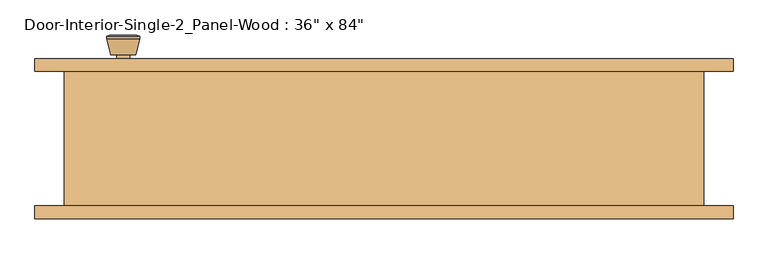
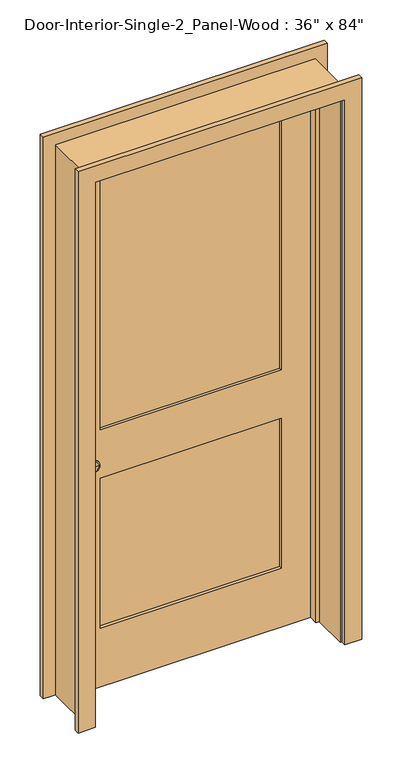
"""IFC4 building model written with IfcOpenShell, lengths in millimetres: door geometry."""

import ifcopenshell
import ifcopenshell.guid

model = None  # the IFC model being written
_history = None  # IfcOwnerHistory: only IFC2X3 demands one
_inside = {}  # id of a spatial element -> (the spatial element, [elements in it])
_under = {}  # id of a project, library or spatial element -> (it, [spatial elements below it])
_declared = {}  # id of a project -> (the project, [libraries it declares])
_typed = {}  # id of a type object -> (the type object, [elements of that type])
_made_of = {}  # id of a material, layer set ... -> (it, [elements and type objects made of it])


def new_model(schema):
    """Start an empty IFC model of exactly this schema.

    Asked for "IFC4X3", IfcOpenShell would pick the latest addendum, in which some entities
    have other attributes; the version numbers below select the first issue.
    IFC2X3 requires an IfcOwnerHistory on every rooted entity: one is made here for all.
    """
    global model, _history
    if schema == "IFC4X3":
        model = ifcopenshell.file(schema_version=(4, 3, 0, 0))
    else:
        model = ifcopenshell.file(schema=schema)
    _inside.clear()
    _under.clear()
    _declared.clear()
    _typed.clear()
    _made_of.clear()
    _history = None
    if model.schema == "IFC2X3":
        org = make("IfcOrganization", Name="unknown")
        user = make(
            "IfcPersonAndOrganization",
            ThePerson=make("IfcPerson", FamilyName="unknown"),
            TheOrganization=org,
        )
        app = make(
            "IfcApplication",
            ApplicationDeveloper=org,
            Version="unknown",
            ApplicationFullName="unknown",
            ApplicationIdentifier="unknown",
        )
        _history = make(
            "IfcOwnerHistory",
            OwningUser=user,
            OwningApplication=app,
            ChangeAction="ADDED",
            CreationDate=0,
        )
    return model


def make(cls, **values):
    """One entity of the class cls with the attributes given. An attribute that is None is left unset."""
    return model.create_entity(
        cls, **{name: value for name, value in values.items() if value is not None}
    )


def rooted(cls, **values):
    """An entity with a GlobalId (a new one), such as an element, a storey or a relation."""
    return make(cls, GlobalId=ifcopenshell.guid.new(), OwnerHistory=_history, **values)


def si_unit(unit_type, name, prefix=None):
    """IfcSIUnit, for example si_unit("LENGTHUNIT", "METRE", prefix="MILLI")."""
    return make("IfcSIUnit", UnitType=unit_type, Prefix=prefix, Name=name)


def assignment(units):
    """IfcUnitAssignment: the units of a project."""
    return None if units is None else make("IfcUnitAssignment", Units=units)


def point(xyz):
    """IfcCartesianPoint."""
    return None if xyz is None else make("IfcCartesianPoint", Coordinates=xyz)


def direction(xyz):
    """IfcDirection."""
    return None if xyz is None else make("IfcDirection", DirectionRatios=xyz)


def frame(location, z_axis=None, x_axis=None):
    """IfcAxis2Placement3D, a coordinate frame: its origin and axes. An axis left out is left unset."""
    return make(
        "IfcAxis2Placement3D",
        Location=point(location),
        Axis=direction(z_axis),
        RefDirection=direction(x_axis),
    )


def frame_2d(location, x_axis=None):
    """IfcAxis2Placement2D, a coordinate frame in the plane: its origin and x axis."""
    return make(
        "IfcAxis2Placement2D", Location=point(location), RefDirection=direction(x_axis)
    )


def origin():
    """The frame at (0, 0, 0) with its axes left unset."""
    return frame((0.0, 0.0, 0.0))


def place(relative_to, where):
    """IfcLocalPlacement: puts the frame where relative to a parent placement (None: the world)."""
    return make(
        "IfcLocalPlacement", PlacementRelTo=relative_to, RelativePlacement=where
    )


def context(
    kind, dimensions, precision=None, world=None, true_north=None, identifier=None
):
    """IfcGeometricRepresentationContext, for example the 3D "Model" context."""
    return make(
        "IfcGeometricRepresentationContext",
        ContextIdentifier=identifier,
        ContextType=kind,
        CoordinateSpaceDimension=dimensions,
        Precision=precision,
        WorldCoordinateSystem=world,
        TrueNorth=true_north,
    )


def project(units=None, contexts=None):
    """IfcProject with its units and contexts."""
    return rooted(
        "IfcProject",
        Name="project",
        RepresentationContexts=contexts,
        UnitsInContext=assignment(units),
    )


def spatial(cls, under=None, at=None, **own):
    """A site, building, storey or space (cls), placed at a placement, below another one or the project."""
    s = rooted(cls, ObjectPlacement=at, **own)
    if under is not None:
        _under.setdefault(under.id(), (under, []))[1].append(s)
    return s


def polyline(points):
    """IfcPolyline through the points."""
    return make("IfcPolyline", Points=[point(p) for p in points])


def circle_curve(where, radius):
    """IfcCircle in the frame where."""
    return make("IfcCircle", Position=where, Radius=radius)


def trimmed(basis, trim1, trim2, sense, master):
    """IfcTrimmedCurve: the piece of a basis curve between two trims."""
    return make(
        "IfcTrimmedCurve",
        BasisCurve=basis,
        Trim1=trim1,
        Trim2=trim2,
        SenseAgreement=sense,
        MasterRepresentation=master,
    )


def segment(curve, same_sense, transition):
    """IfcCompositeCurveSegment."""
    return make(
        "IfcCompositeCurveSegment",
        Transition=transition,
        SameSense=same_sense,
        ParentCurve=curve,
    )


def composite_curve(segments, self_intersect=None):
    """IfcCompositeCurve: segments joined end to end."""
    return make("IfcCompositeCurve", Segments=segments, SelfIntersect=self_intersect)


def outline(outer, holes=None, kind="AREA"):
    """IfcArbitraryClosedProfileDef: a profile drawn as a closed curve; with holes, ...WithVoids."""
    if holes is None:
        return make("IfcArbitraryClosedProfileDef", ProfileType=kind, OuterCurve=outer)
    return make(
        "IfcArbitraryProfileDefWithVoids",
        ProfileType=kind,
        OuterCurve=outer,
        InnerCurves=holes,
    )


def extrude(swept, where, along, depth):
    """IfcExtrudedAreaSolid: the profile swept, set in the frame where, extruded along a direction by depth."""
    return make(
        "IfcExtrudedAreaSolid",
        SweptArea=swept,
        Position=where,
        ExtrudedDirection=direction(along),
        Depth=depth,
    )


def faces_of(points, faces, orient=None, outer=None):
    """IfcFace entities. A face is a list of loops; a loop is a list of indices into points, from 0.

    orient and outer hold one flag for each loop. By default every Orientation is true, the
    first loop of a face is its IfcFaceOuterBound and the others are IfcFaceBound.
    """
    made = []
    for i, loops in enumerate(faces):
        bounds = []
        for j, loop in enumerate(loops):
            is_outer = j == 0 if outer is None else outer[i][j]
            bounds.append(
                make(
                    "IfcFaceOuterBound" if is_outer else "IfcFaceBound",
                    Bound=make("IfcPolyLoop", Polygon=[points[k] for k in loop]),
                    Orientation=True if orient is None else orient[i][j],
                )
            )
        made.append(make("IfcFace", Bounds=bounds))
    return made


def faceted_brep(points, faces, orient=None, outer=None, voids=None):
    """IfcFacetedBrep: a solid bounded by flat faces; with voids (closed shells), ...WithVoids."""
    shared = [point(p) for p in points]
    hull = make("IfcClosedShell", CfsFaces=faces_of(shared, faces, orient, outer))
    if voids is None:
        return make("IfcFacetedBrep", Outer=hull)
    return make(
        "IfcFacetedBrepWithVoids",
        Outer=hull,
        Voids=[
            make(cls, CfsFaces=faces_of(shared, fs, o, b)) for cls, fs, o, b in voids
        ],
    )


def shape(context_of_items, identifier, shape_type, items):
    """IfcShapeRepresentation: the items that make up one representation, for example the "Body"."""
    return make(
        "IfcShapeRepresentation",
        ContextOfItems=context_of_items,
        RepresentationIdentifier=identifier,
        RepresentationType=shape_type,
        Items=items,
    )


def source(mapping_origin, context_of_items, identifier, shape_type, items):
    """IfcRepresentationMap: a shape defined once, which mapped items show again and again."""
    return make(
        "IfcRepresentationMap",
        MappingOrigin=mapping_origin,
        MappedRepresentation=shape(context_of_items, identifier, shape_type, items),
    )


def transform(
    local_origin,
    x_axis=None,
    y_axis=None,
    z_axis=None,
    scale=None,
    scale2=None,
    scale3=None,
    uniform=True,
):
    """IfcCartesianTransformationOperator3D, or its non-uniform kind. x_axis, y_axis, z_axis: its Axis1, 2, 3."""
    if uniform:
        return make(
            "IfcCartesianTransformationOperator3D",
            Axis1=direction(x_axis),
            Axis2=direction(y_axis),
            LocalOrigin=point(local_origin),
            Scale=scale,
            Axis3=direction(z_axis),
        )
    return make(
        "IfcCartesianTransformationOperator3DnonUniform",
        Axis1=direction(x_axis),
        Axis2=direction(y_axis),
        LocalOrigin=point(local_origin),
        Scale=scale,
        Axis3=direction(z_axis),
        Scale2=scale2,
        Scale3=scale3,
    )


def mapped(mapping_source, mapping_target):
    """IfcMappedItem: shows the shape of a source again, moved by a transform."""
    return make(
        "IfcMappedItem", MappingSource=mapping_source, MappingTarget=mapping_target
    )


def made_of(thing, what):
    """Note that an element or type object is made of a material, layer set ...; save() writes the relation."""
    if what is not None:
        _made_of.setdefault(what.id(), (what, []))[1].append(thing)
    return thing


def element(
    cls,
    number,
    at=None,
    inside=None,
    cuts=None,
    type_object=None,
    material=None,
    context=None,
    identifier="Body",
    shape_type=None,
    held_by="IfcProductDefinitionShape",
    body=None,
    shapes=None,
    **own,
):
    """One element of the class cls, such as IfcWall. Its Tag is "e" and its number.

    at: its placement. inside: the storey or other place that contains it. cuts: it is an
    opening in that element (IfcRelVoidsElement). A single representation is given by context,
    identifier, shape_type and body (its items); several are given by shapes. held_by: the class
    of the entity that holds the representations. save() writes the other relations.
    """
    e = rooted(cls, Tag="e%d" % number, ObjectPlacement=at, **own)
    if body is not None:
        shapes = [shape(context, identifier, shape_type, body)]
    if shapes is not None:
        e.Representation = make(held_by, Representations=shapes)
    if inside is not None:
        _inside.setdefault(inside.id(), (inside, []))[1].append(e)
    if cuts is not None:
        rooted(
            "IfcRelVoidsElement", RelatingBuildingElement=cuts, RelatedOpeningElement=e
        )
    if type_object is not None:
        _typed.setdefault(type_object.id(), (type_object, []))[1].append(e)
    return made_of(e, material)


def aggregate(whole, parts):
    """IfcRelAggregates: a whole, such as a stair, and the parts it consists of."""
    return rooted("IfcRelAggregates", RelatingObject=whole, RelatedObjects=parts)


def save(model, path):
    """Write the relations noted so far, then the file.

    IfcRelAggregates (storeys below a building ...), IfcRelContainedInSpatialStructure (elements
    in a storey), IfcRelDefinesByType, IfcRelAssociatesMaterial and IfcRelDeclares: one each for
    every whole, place, type object, material and project.
    """
    for whole, parts in _under.values():
        aggregate(whole, parts)
    for where, things in _inside.values():
        rooted(
            "IfcRelContainedInSpatialStructure",
            RelatedElements=things,
            RelatingStructure=where,
        )
    for kind, things in _typed.values():
        rooted("IfcRelDefinesByType", RelatedObjects=things, RelatingType=kind)
    for what, things in _made_of.values():
        rooted("IfcRelAssociatesMaterial", RelatedObjects=things, RelatingMaterial=what)
    for by, libraries in _declared.values():
        rooted("IfcRelDeclares", RelatingContext=by, RelatedDefinitions=libraries)
    model.write(path)


def plane_surface(at):
    """IfcPlane: the flat surface through the origin of the frame at, square to its z axis."""
    return make("IfcPlane", Position=at)


def cylinder_surface(at, radius):
    """IfcCylindricalSurface: all points at the distance radius from the z axis of the frame at."""
    return make("IfcCylindricalSurface", Position=at, Radius=radius)


def revolved_surface(curve, axis_point, axis_direction):
    """IfcSurfaceOfRevolution: the curve turned about the line through axis_point along axis_direction."""
    return make(
        "IfcSurfaceOfRevolution",
        SweptCurve=make("IfcArbitraryOpenProfileDef", ProfileType="CURVE", Curve=curve),
        AxisPosition=make("IfcAxis1Placement", Location=point(axis_point), Axis=direction(axis_direction)),
    )


def advanced_brep(points, edges, surfaces, faces):
    """IfcAdvancedBrep: a solid bounded by faces that lie on surfaces and meet in shared edges.

    An edge is (start, end): straight between two places in points (the first is 0);
    or (start, end, curve); or (start, end, curve, False) where it runs against its curve.
    A face is (place in surfaces, loops), or (place, loops, False) where it looks against
    its surface's normal. A loop lists edges by number (the first is 1), with a minus sign
    where the edge is run from its end to its start. The first loop is the outer one.
    """
    corners = [point(p) for p in points]
    vertices = [make("IfcVertexPoint", VertexGeometry=c) for c in corners]
    made = []
    for start, end, *more in edges:
        made.append(
            make(
                "IfcEdgeCurve",
                EdgeStart=vertices[start],
                EdgeEnd=vertices[end],
                EdgeGeometry=more[0] if more else make("IfcPolyline", Points=[corners[start], corners[end]]),
                SameSense=more[1] if len(more) > 1 else True,
            )
        )
    hull = []
    for where, loops, *sense in faces:
        bounds = []
        for j, loop in enumerate(loops):
            ring = [make("IfcOrientedEdge", EdgeElement=made[abs(k) - 1], Orientation=k > 0) for k in loop]
            bounds.append(
                make(
                    "IfcFaceOuterBound" if j == 0 else "IfcFaceBound",
                    Bound=make("IfcEdgeLoop", EdgeList=ring),
                    Orientation=True,
                )
            )
        hull.append(make("IfcAdvancedFace", Bounds=bounds, FaceSurface=surfaces[where], SameSense=sense[0] if sense else True))
    return make("IfcAdvancedBrep", Outer=make("IfcClosedShell", CfsFaces=hull))


def door_6f959a6d(model_context):
    return source(origin(), model_context, "Body", "SolidModel", [
        advanced_brep(
        [(-393.7, 57.5, 914.4), (-383.7, 57.5, 914.4), (-403.7, 57.5, 914.4), (-373.2241324, 8.5, 914.4), (-393.7, 8.5, 914.4), (-414.1758676, 8.5, 914.4), (-368.7, 10.3278681, 914.4), (-418.7, 10.3278681, 914.4), (-368.7, 13.7915463, 914.4), (-418.7, 13.7915463, 914.4), (-375.063764, 38.5, 914.4), (-412.336236, 38.5, 914.4), (-383.7, 38.5, 914.4), (-403.7, 38.5, 914.4)],
        [
            (0, 1),
            (1, 2, circle_curve(frame((-393.7, 57.5, 914.4), z_axis=(0.0, 1.0, 0.0), x_axis=(-1.0, 0.0, 0.0)), 10.0)),
            (2, 0),
            (2, 1, circle_curve(frame((-393.7, 57.5, 914.4), z_axis=(0.0, 1.0, 0.0), x_axis=(-1.0, 0.0, 0.0)), 10.0)),
            (3, 4),
            (4, 5),
            (5, 3, circle_curve(frame((-393.7, 8.5, 914.4), z_axis=(0.0, -1.0, 0.0), x_axis=(-1.0, 0.0, 0.0)), 20.4758676)),
            (3, 5, circle_curve(frame((-393.7, 8.5, 914.4), z_axis=(0.0, -1.0, 0.0), x_axis=(-1.0, 0.0, 0.0)), 20.4758676)),
            (6, 3),
            (5, 7),
            (7, 6, circle_curve(frame((-393.7, 10.3278681, 914.4), z_axis=(0.0, -1.0, 0.0), x_axis=(-1.0, 0.0, 0.0)), 25.0)),
            (6, 7, circle_curve(frame((-393.7, 10.3278681, 914.4), z_axis=(0.0, -1.0, 0.0), x_axis=(-1.0, 0.0, 0.0)), 25.0)),
            (8, 6),
            (7, 9),
            (9, 8, circle_curve(frame((-393.7, 13.7915463, 914.4), z_axis=(0.0, -1.0, 0.0), x_axis=(-1.0, 0.0, 0.0)), 25.0)),
            (8, 9, circle_curve(frame((-393.7, 13.7915463, 914.4), z_axis=(0.0, -1.0, 0.0), x_axis=(-1.0, 0.0, 0.0)), 25.0)),
            (10, 8),
            (9, 11),
            (11, 10, circle_curve(frame((-393.7, 38.5, 914.4), z_axis=(0.0, -1.0, 0.0), x_axis=(-1.0, 0.0, 0.0)), 18.636236)),
            (10, 11, circle_curve(frame((-393.7, 38.5, 914.4), z_axis=(0.0, -1.0, 0.0), x_axis=(-1.0, 0.0, 0.0)), 18.636236)),
            (12, 10),
            (11, 13),
            (13, 12, circle_curve(frame((-393.7, 38.5, 914.4), z_axis=(0.0, -1.0, 0.0), x_axis=(-1.0, 0.0, 0.0)), 10.0)),
            (12, 13, circle_curve(frame((-393.7, 38.5, 914.4), z_axis=(0.0, -1.0, 0.0), x_axis=(-1.0, 0.0, 0.0)), 10.0)),
            (1, 12),
            (13, 2),
        ],
        [
            plane_surface(frame((-393.7, 57.5, 914.4), z_axis=(0.0, 1.0, 0.0), x_axis=(-1.0, 0.0, 0.0))),
            plane_surface(frame((-393.7, 8.5, 914.4), z_axis=(0.0, -1.0, 0.0), x_axis=(-1.0, 0.0, 0.0))),
            revolved_surface(polyline([(-414.1758676, 8.5, 914.4), (-418.7, 10.3278681, 914.4)]), (-393.7, 57.5, 914.4), (0.0, 1.0, 0.0)),
            cylinder_surface(frame((-393.7, 57.5, 914.4), z_axis=(0.0, 1.0, 0.0), x_axis=(-1.0, 0.0, 0.0)), 25.0),
            revolved_surface(polyline([(-418.7, 13.7915463, 914.4), (-412.336236, 38.5, 914.4)]), (-393.7, 57.5, 914.4), (0.0, 1.0, 0.0)),
            plane_surface(frame((-393.7, 38.5, 914.4), z_axis=(0.0, 1.0, 0.0), x_axis=(-1.0, 0.0, 0.0))),
            cylinder_surface(frame((-393.7, 57.5, 914.4), z_axis=(0.0, 1.0, 0.0), x_axis=(-1.0, 0.0, 0.0)), 10.0),
        ],
        [
            (0, [[1, 2, 3]]),
            (0, [[-3, 4, -1]]),
            (1, [[5, 6, 7]]),
            (1, [[-6, -5, 8]]),
            (2, [[9, -7, 10, 11]]),
            (2, [[-10, -8, -9, 12]]),
            (3, [[13, -11, 14, 15]]),
            (3, [[-14, -12, -13, 16]]),
            (4, [[17, -15, 18, 19]]),
            (4, [[-18, -16, -17, 20]]),
            (5, [[21, -19, 22, 23]]),
            (5, [[-22, -20, -21, 24]]),
            (6, [[25, -23, 26, -2]]),
            (6, [[-26, -24, -25, -4]]),
        ],
    ),
        extrude(outline(composite_curve([segment(trimmed(circle_curve(frame_2d((914.4, -393.7)), 30.0), [point((914.4, -423.7))], [point((914.4, -363.7))], False, "CARTESIAN"), True, "CONTINUOUS"), segment(trimmed(circle_curve(frame_2d((914.4, -393.7)), 30.0), [point((914.4, -363.7))], [point((914.4, -423.7))], False, "CARTESIAN"), True, "CONTINUOUS")], self_intersect=False)), frame((0.0, 57.5, 0.0), z_axis=(0.0, 1.0, 0.0), x_axis=(0.0, 0.0, 1.0)), (0.0, 0.0, 1.0), 6.0),
        advanced_brep(
        [(-393.7, 104.425, 914.4), (-403.7, 104.425, 914.4), (-383.7, 104.425, 914.4), (-373.2241324, 153.425, 914.4), (-414.1758676, 153.425, 914.4), (-393.7, 153.425, 914.4), (-368.7, 151.5971319, 914.4), (-418.7, 151.5971319, 914.4), (-368.7, 148.1334537, 914.4), (-418.7, 148.1334537, 914.4), (-375.063764, 123.425, 914.4), (-412.336236, 123.425, 914.4), (-383.7, 123.425, 914.4), (-403.7, 123.425, 914.4)],
        [
            (0, 1),
            (1, 2, circle_curve(frame((-393.7, 104.425, 914.4), z_axis=(0.0, -1.0, 0.0), x_axis=(-1.0, 0.0, 0.0)), 10.0)),
            (2, 0),
            (2, 1, circle_curve(frame((-393.7, 104.425, 914.4), z_axis=(0.0, -1.0, 0.0), x_axis=(-1.0, 0.0, 0.0)), 10.0)),
            (3, 4, circle_curve(frame((-393.7, 153.425, 914.4), z_axis=(0.0, 1.0, 0.0), x_axis=(-1.0, 0.0, 0.0)), 20.4758676)),
            (4, 5),
            (5, 3),
            (4, 3, circle_curve(frame((-393.7, 153.425, 914.4), z_axis=(0.0, 1.0, 0.0), x_axis=(-1.0, 0.0, 0.0)), 20.4758676)),
            (6, 7, circle_curve(frame((-393.7, 151.5971319, 914.4), z_axis=(0.0, 1.0, 0.0), x_axis=(-1.0, 0.0, 0.0)), 25.0)),
            (7, 4),
            (3, 6),
            (7, 6, circle_curve(frame((-393.7, 151.5971319, 914.4), z_axis=(0.0, 1.0, 0.0), x_axis=(-1.0, 0.0, 0.0)), 25.0)),
            (8, 9, circle_curve(frame((-393.7, 148.1334537, 914.4), z_axis=(0.0, 1.0, 0.0), x_axis=(-1.0, 0.0, 0.0)), 25.0)),
            (9, 7),
            (6, 8),
            (9, 8, circle_curve(frame((-393.7, 148.1334537, 914.4), z_axis=(0.0, 1.0, 0.0), x_axis=(-1.0, 0.0, 0.0)), 25.0)),
            (10, 11, circle_curve(frame((-393.7, 123.425, 914.4), z_axis=(0.0, 1.0, 0.0), x_axis=(-1.0, 0.0, 0.0)), 18.636236)),
            (11, 9),
            (8, 10),
            (11, 10, circle_curve(frame((-393.7, 123.425, 914.4), z_axis=(0.0, 1.0, 0.0), x_axis=(-1.0, 0.0, 0.0)), 18.636236)),
            (12, 13, circle_curve(frame((-393.7, 123.425, 914.4), z_axis=(0.0, 1.0, 0.0), x_axis=(-1.0, 0.0, 0.0)), 10.0)),
            (13, 11),
            (10, 12),
            (13, 12, circle_curve(frame((-393.7, 123.425, 914.4), z_axis=(0.0, 1.0, 0.0), x_axis=(-1.0, 0.0, 0.0)), 10.0)),
            (1, 13),
            (12, 2),
        ],
        [
            plane_surface(frame((-393.7, 104.425, 914.4), z_axis=(0.0, -1.0, 0.0), x_axis=(-1.0, 0.0, 0.0))),
            plane_surface(frame((-393.7, 153.425, 914.4), z_axis=(0.0, 1.0, 0.0), x_axis=(-1.0, 0.0, 0.0))),
            revolved_surface(polyline([(-414.1758676, 153.425, 914.4), (-418.7, 151.5971319, 914.4)]), (-393.7, 104.425, 914.4), (0.0, -1.0, 0.0)),
            cylinder_surface(frame((-393.7, 104.425, 914.4), z_axis=(0.0, -1.0, 0.0), x_axis=(-1.0, 0.0, 0.0)), 25.0),
            revolved_surface(polyline([(-418.7, 148.1334537, 914.4), (-412.336236, 123.425, 914.4)]), (-393.7, 104.425, 914.4), (0.0, -1.0, 0.0)),
            plane_surface(frame((-393.7, 123.425, 914.4), z_axis=(0.0, -1.0, 0.0), x_axis=(-1.0, 0.0, 0.0))),
            cylinder_surface(frame((-393.7, 104.425, 914.4), z_axis=(0.0, -1.0, 0.0), x_axis=(-1.0, 0.0, 0.0)), 10.0),
        ],
        [
            (0, [[1, 2, 3]]),
            (0, [[-3, 4, -1]]),
            (1, [[5, 6, 7]]),
            (1, [[8, -7, -6]]),
            (2, [[9, 10, -5, 11]]),
            (2, [[12, -11, -8, -10]]),
            (3, [[13, 14, -9, 15]]),
            (3, [[16, -15, -12, -14]]),
            (4, [[17, 18, -13, 19]]),
            (4, [[20, -19, -16, -18]]),
            (5, [[21, 22, -17, 23]]),
            (5, [[24, -23, -20, -22]]),
            (6, [[-2, 25, -21, 26]]),
            (6, [[-4, -26, -24, -25]]),
        ],
    ),
        extrude(outline(composite_curve([segment(trimmed(circle_curve(frame_2d((914.4, -393.7)), 30.0), [point((914.4, -423.7))], [point((914.4, -363.7))], False, "CARTESIAN"), True, "CONTINUOUS"), segment(trimmed(circle_curve(frame_2d((914.4, -393.7)), 30.0), [point((914.4, -363.7))], [point((914.4, -423.7))], False, "CARTESIAN"), True, "CONTINUOUS")], self_intersect=False)), frame((0.0, 98.425, 0.0), z_axis=(0.0, 1.0, 0.0), x_axis=(0.0, 0.0, 1.0)), (0.0, 0.0, 1.0), 6.0),
        extrude(outline(polyline([(336.55, 75.1416667), (-336.55, 75.1416667), (-336.55, 86.7833333), (336.55, 86.7833333), (336.55, 75.1416667)])), frame((0.0, 0.0, 1009.65), z_axis=(0.0, 0.0, 1.0), x_axis=(1.0, 0.0, 0.0)), (0.0, 0.0, 1.0), 1004.8875),
        extrude(outline(polyline([(336.55, 75.1416667), (-336.55, 75.1416667), (-336.55, 86.7833333), (336.55, 86.7833333), (336.55, 75.1416667)])), frame((0.0, 0.0, 231.775), z_axis=(0.0, 0.0, 1.0), x_axis=(1.0, 0.0, 0.0)), (0.0, 0.0, 1.0), 587.375),
        extrude(outline(polyline([(2133.6, -457.2), (0.0, -457.2), (0.0, 457.2), (2133.6, 457.2), (2133.6, -457.2)]), holes=[polyline([(2014.5375, -336.55), (2014.5375, 336.55), (1009.65, 336.55), (1009.65, -336.55), (2014.5375, -336.55)]), polyline([(819.15, -336.55), (819.15, 336.55), (231.775, 336.55), (231.775, -336.55), (819.15, -336.55)])]), frame((0.0, 63.5, 0.0), z_axis=(0.0, 1.0, 0.0), x_axis=(0.0, 0.0, 1.0)), (0.0, 0.0, 1.0), 34.925),
        faceted_brep([(482.6, 98.425, 0.0), (482.6, -104.775, 0.0), (457.2, -104.775, 0.0), (457.2, 28.575, 0.0), (444.5, 28.575, 0.0), (444.5, 63.5, 0.0), (457.2, 63.5, 0.0), (457.2, 98.425, 0.0), (482.6, 98.425, 2159.0), (482.6, -104.775, 2159.0), (-482.6, -104.775, 2159.0), (-482.6, -104.775, 0.0), (-457.2, -104.775, 0.0), (-457.2, -104.775, 2133.6), (457.2, -104.775, 2133.6), (457.2, 28.575, 2133.6), (-457.2, 28.575, 2133.6), (-457.2, 28.575, 0.0), (-444.5, 28.575, 0.0), (-444.5, 28.575, 2120.9), (444.5, 28.575, 2120.9), (444.5, 63.5, 2120.9), (-444.5, 63.5, 2120.9), (-444.5, 63.5, 0.0), (-457.2, 63.5, 0.0), (-457.2, 63.5, 2133.6), (457.2, 63.5, 2133.6), (457.2, 98.425, 2133.6), (-457.2, 98.425, 2133.6), (-457.2, 98.425, 0.0), (-482.6, 98.425, 0.0), (-482.6, 98.425, 2159.0)], [[[0, 1, 2, 3, 4, 5, 6, 7]], [[1, 0, 8, 9]], [[2, 1, 9, 10, 11, 12, 13, 14]], [[3, 2, 14, 15]], [[4, 3, 15, 16, 17, 18, 19, 20]], [[5, 4, 20, 21]], [[6, 5, 21, 22, 23, 24, 25, 26]], [[7, 6, 26, 27]], [[0, 7, 27, 28, 29, 30, 31, 8]], [[9, 8, 31, 10]], [[15, 14, 13, 16]], [[21, 20, 19, 22]], [[27, 26, 25, 28]], [[30, 29, 24, 23, 18, 17, 12, 11]], [[10, 31, 30, 11]], [[16, 13, 12, 17]], [[22, 19, 18, 23]], [[28, 25, 24, 29]]]),
        extrude(outline(polyline([(0.0, 463.55), (0.0, 527.05), (2203.45, 527.05), (2203.45, -527.05), (0.0, -527.05), (0.0, -463.55), (2139.95, -463.55), (2139.95, 463.55), (0.0, 463.55)])), frame((0.0, -123.825, 0.0), z_axis=(0.0, 1.0, 0.0), x_axis=(0.0, 0.0, 1.0)), (0.0, 0.0, 1.0), 19.05),
        extrude(outline(polyline([(0.0, 463.55), (0.0, 527.05), (2203.45, 527.05), (2203.45, -527.05), (0.0, -527.05), (0.0, -463.55), (2139.95, -463.55), (2139.95, 463.55), (0.0, 463.55)])), frame((0.0, 98.425, 0.0), z_axis=(0.0, 1.0, 0.0), x_axis=(0.0, 0.0, 1.0)), (0.0, 0.0, 1.0), 19.05),
    ])


if __name__ == "__main__":
    model = new_model("IFC4")
    model_context = context("Model", 3, world=origin())
    ifc_project = project(units=[si_unit("LENGTHUNIT", "METRE", prefix="MILLI")], contexts=[model_context])
    site = spatial("IfcSite", under=ifc_project)
    building = spatial("IfcBuilding", under=site)
    placement = place(None, origin())
    door_shape = door_6f959a6d(model_context)
    element("IfcDoor", 1, ObjectType="Door-Interior-Single-2_Panel-Wood : 36\" x 84\"", at=placement, inside=building, context=model_context, shape_type="MappedRepresentation", body=[
        mapped(door_shape, transform((0.0, 0.0, 0.0), x_axis=(1.0, 0.0, 0.0), y_axis=(0.0, 1.0, 0.0), z_axis=(0.0, 0.0, 1.0))),
    ])
    save(model, "model.ifc")

# Revit data of these elements
# Type "Door-Interior-Single-2_Panel-Wood : 36\" x 84\""
#   Type Mark = "17"
#   Assembly Code = "C1020300"
#   Analytic Construction = "Wooden"
#   Top Rail = 0' - 4 11/16"
#   Thickness = 0' - 1 3/8"
#   Thermal Resistance (R) = 2.5876 (h·ft²·°F)/BTU
#   Swing Angle [instance default] = 90.00°
#   Stiles = 0' - 4 3/4"
#   Rough Width = 3' - 2"
#   Rough Height = 7' - 1"
#   Lock Rail = 0' - 7 1/2"
#   Height = 7' - 0"
#   Width = 3' - 0"
#   Heat Transfer Coefficient (U) = 0.3865 BTU/(h·ft²·°F)
#   Bottom Rail = 0' - 9 1/8"
#   Function = 0
#   Trim Material = Cherry
#   Panel Material = Cherry
#   Frame Material = Cherry
#   Door Handle Material = Aluminum
#   Visual Light Transmittance = 0
#   Solar Heat Gain Coefficient = 0
#   Wall Closure = (empty or 0)
#   Function = (empty or 0)
# Element 1 (IfcDoor, "Door-Interior-Single-2_Panel-Wood : 36\" x 84\"")
#   Materials on its faces: "Cherry", "Aluminum"
# Materials
#   "Cherry": class "Wood", colour RGB 157 77 38, transparency 0, Description = "Prunus Serotina", Cost = 0
#   "Aluminum": class "Metal", colour RGB 120 120 120, transparency 0, Description = "Aluminum 6061", Cost = 0
